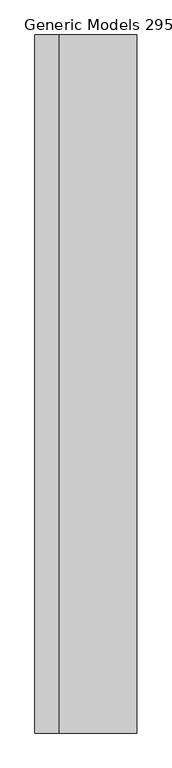
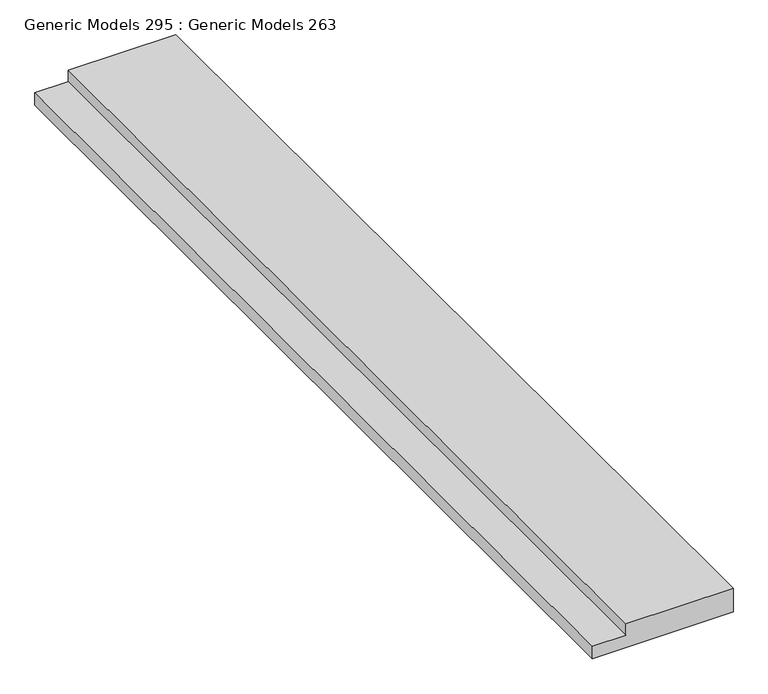
"""IFC4 building model written with IfcOpenShell, lengths in millimetres: proxy geometry, Generic Models 295 : Generic Models 263."""

import ifcopenshell
import ifcopenshell.guid

model = None  # the IFC model being written
_history = None  # IfcOwnerHistory: only IFC2X3 demands one
_inside = {}  # id of a spatial element -> (the spatial element, [elements in it])
_under = {}  # id of a project, library or spatial element -> (it, [spatial elements below it])
_declared = {}  # id of a project -> (the project, [libraries it declares])
_typed = {}  # id of a type object -> (the type object, [elements of that type])
_made_of = {}  # id of a material, layer set ... -> (it, [elements and type objects made of it])


def new_model(schema):
    """Start an empty IFC model of exactly this schema.

    Asked for "IFC4X3", IfcOpenShell would pick the latest addendum, in which some entities
    have other attributes; the version numbers below select the first issue.
    IFC2X3 requires an IfcOwnerHistory on every rooted entity: one is made here for all.
    """
    global model, _history
    if schema == "IFC4X3":
        model = ifcopenshell.file(schema_version=(4, 3, 0, 0))
    else:
        model = ifcopenshell.file(schema=schema)
    _inside.clear()
    _under.clear()
    _declared.clear()
    _typed.clear()
    _made_of.clear()
    _history = None
    if model.schema == "IFC2X3":
        org = make("IfcOrganization", Name="unknown")
        user = make(
            "IfcPersonAndOrganization",
            ThePerson=make("IfcPerson", FamilyName="unknown"),
            TheOrganization=org,
        )
        app = make(
            "IfcApplication",
            ApplicationDeveloper=org,
            Version="unknown",
            ApplicationFullName="unknown",
            ApplicationIdentifier="unknown",
        )
        _history = make(
            "IfcOwnerHistory",
            OwningUser=user,
            OwningApplication=app,
            ChangeAction="ADDED",
            CreationDate=0,
        )
    return model


def make(cls, **values):
    """One entity of the class cls with the attributes given. An attribute that is None is left unset."""
    return model.create_entity(
        cls, **{name: value for name, value in values.items() if value is not None}
    )


def rooted(cls, **values):
    """An entity with a GlobalId (a new one), such as an element, a storey or a relation."""
    return make(cls, GlobalId=ifcopenshell.guid.new(), OwnerHistory=_history, **values)


def si_unit(unit_type, name, prefix=None):
    """IfcSIUnit, for example si_unit("LENGTHUNIT", "METRE", prefix="MILLI")."""
    return make("IfcSIUnit", UnitType=unit_type, Prefix=prefix, Name=name)


def assignment(units):
    """IfcUnitAssignment: the units of a project."""
    return None if units is None else make("IfcUnitAssignment", Units=units)


def point(xyz):
    """IfcCartesianPoint."""
    return None if xyz is None else make("IfcCartesianPoint", Coordinates=xyz)


def direction(xyz):
    """IfcDirection."""
    return None if xyz is None else make("IfcDirection", DirectionRatios=xyz)


def frame(location, z_axis=None, x_axis=None):
    """IfcAxis2Placement3D, a coordinate frame: its origin and axes. An axis left out is left unset."""
    return make(
        "IfcAxis2Placement3D",
        Location=point(location),
        Axis=direction(z_axis),
        RefDirection=direction(x_axis),
    )


def origin():
    """The frame at (0, 0, 0) with its axes left unset."""
    return frame((0.0, 0.0, 0.0))


def place(relative_to, where):
    """IfcLocalPlacement: puts the frame where relative to a parent placement (None: the world)."""
    return make(
        "IfcLocalPlacement", PlacementRelTo=relative_to, RelativePlacement=where
    )


def context(
    kind, dimensions, precision=None, world=None, true_north=None, identifier=None
):
    """IfcGeometricRepresentationContext, for example the 3D "Model" context."""
    return make(
        "IfcGeometricRepresentationContext",
        ContextIdentifier=identifier,
        ContextType=kind,
        CoordinateSpaceDimension=dimensions,
        Precision=precision,
        WorldCoordinateSystem=world,
        TrueNorth=true_north,
    )


def project(units=None, contexts=None):
    """IfcProject with its units and contexts."""
    return rooted(
        "IfcProject",
        Name="project",
        RepresentationContexts=contexts,
        UnitsInContext=assignment(units),
    )


def spatial(cls, under=None, at=None, **own):
    """A site, building, storey or space (cls), placed at a placement, below another one or the project."""
    s = rooted(cls, ObjectPlacement=at, **own)
    if under is not None:
        _under.setdefault(under.id(), (under, []))[1].append(s)
    return s


def polyline(points):
    """IfcPolyline through the points."""
    return make("IfcPolyline", Points=[point(p) for p in points])


def outline(outer, holes=None, kind="AREA"):
    """IfcArbitraryClosedProfileDef: a profile drawn as a closed curve; with holes, ...WithVoids."""
    if holes is None:
        return make("IfcArbitraryClosedProfileDef", ProfileType=kind, OuterCurve=outer)
    return make(
        "IfcArbitraryProfileDefWithVoids",
        ProfileType=kind,
        OuterCurve=outer,
        InnerCurves=holes,
    )


def extrude(swept, where, along, depth):
    """IfcExtrudedAreaSolid: the profile swept, set in the frame where, extruded along a direction by depth."""
    return make(
        "IfcExtrudedAreaSolid",
        SweptArea=swept,
        Position=where,
        ExtrudedDirection=direction(along),
        Depth=depth,
    )


def shape(context_of_items, identifier, shape_type, items):
    """IfcShapeRepresentation: the items that make up one representation, for example the "Body"."""
    return make(
        "IfcShapeRepresentation",
        ContextOfItems=context_of_items,
        RepresentationIdentifier=identifier,
        RepresentationType=shape_type,
        Items=items,
    )


def source(mapping_origin, context_of_items, identifier, shape_type, items):
    """IfcRepresentationMap: a shape defined once, which mapped items show again and again."""
    return make(
        "IfcRepresentationMap",
        MappingOrigin=mapping_origin,
        MappedRepresentation=shape(context_of_items, identifier, shape_type, items),
    )


def transform(
    local_origin,
    x_axis=None,
    y_axis=None,
    z_axis=None,
    scale=None,
    scale2=None,
    scale3=None,
    uniform=True,
):
    """IfcCartesianTransformationOperator3D, or its non-uniform kind. x_axis, y_axis, z_axis: its Axis1, 2, 3."""
    if uniform:
        return make(
            "IfcCartesianTransformationOperator3D",
            Axis1=direction(x_axis),
            Axis2=direction(y_axis),
            LocalOrigin=point(local_origin),
            Scale=scale,
            Axis3=direction(z_axis),
        )
    return make(
        "IfcCartesianTransformationOperator3DnonUniform",
        Axis1=direction(x_axis),
        Axis2=direction(y_axis),
        LocalOrigin=point(local_origin),
        Scale=scale,
        Axis3=direction(z_axis),
        Scale2=scale2,
        Scale3=scale3,
    )


def mapped(mapping_source, mapping_target):
    """IfcMappedItem: shows the shape of a source again, moved by a transform."""
    return make(
        "IfcMappedItem", MappingSource=mapping_source, MappingTarget=mapping_target
    )


def made_of(thing, what):
    """Note that an element or type object is made of a material, layer set ...; save() writes the relation."""
    if what is not None:
        _made_of.setdefault(what.id(), (what, []))[1].append(thing)
    return thing


def element(
    cls,
    number,
    at=None,
    inside=None,
    cuts=None,
    type_object=None,
    material=None,
    context=None,
    identifier="Body",
    shape_type=None,
    held_by="IfcProductDefinitionShape",
    body=None,
    shapes=None,
    **own,
):
    """One element of the class cls, such as IfcWall. Its Tag is "e" and its number.

    at: its placement. inside: the storey or other place that contains it. cuts: it is an
    opening in that element (IfcRelVoidsElement). A single representation is given by context,
    identifier, shape_type and body (its items); several are given by shapes. held_by: the class
    of the entity that holds the representations. save() writes the other relations.
    """
    e = rooted(cls, Tag="e%d" % number, ObjectPlacement=at, **own)
    if body is not None:
        shapes = [shape(context, identifier, shape_type, body)]
    if shapes is not None:
        e.Representation = make(held_by, Representations=shapes)
    if inside is not None:
        _inside.setdefault(inside.id(), (inside, []))[1].append(e)
    if cuts is not None:
        rooted(
            "IfcRelVoidsElement", RelatingBuildingElement=cuts, RelatedOpeningElement=e
        )
    if type_object is not None:
        _typed.setdefault(type_object.id(), (type_object, []))[1].append(e)
    return made_of(e, material)


def aggregate(whole, parts):
    """IfcRelAggregates: a whole, such as a stair, and the parts it consists of."""
    return rooted("IfcRelAggregates", RelatingObject=whole, RelatedObjects=parts)


def save(model, path):
    """Write the relations noted so far, then the file.

    IfcRelAggregates (storeys below a building ...), IfcRelContainedInSpatialStructure (elements
    in a storey), IfcRelDefinesByType, IfcRelAssociatesMaterial and IfcRelDeclares: one each for
    every whole, place, type object, material and project.
    """
    for whole, parts in _under.values():
        aggregate(whole, parts)
    for where, things in _inside.values():
        rooted(
            "IfcRelContainedInSpatialStructure",
            RelatedElements=things,
            RelatingStructure=where,
        )
    for kind, things in _typed.values():
        rooted("IfcRelDefinesByType", RelatedObjects=things, RelatingType=kind)
    for what, things in _made_of.values():
        rooted("IfcRelAssociatesMaterial", RelatedObjects=things, RelatingMaterial=what)
    for by, libraries in _declared.values():
        rooted("IfcRelDeclares", RelatingContext=by, RelatedDefinitions=libraries)
    model.write(path)


def generic_models_295_generic_models_263_197a9b76(model_context):
    return source(origin(), model_context, "Body", "SweptSolid", [
        extrude(outline(polyline([(-381.0, 92037.1797726), (-381.0, 91579.9797726), (-558.8, 91579.9797726), (-558.8, 93498.3966125), (-215.9, 93498.3966125), (-215.9, 92037.1797726), (-381.0, 92037.1797726)])), frame((0.0, -4692.2809088, 0.0), z_axis=(0.0, 1.0, 0.0), x_axis=(0.0, 0.0, 1.0)), (0.0, 0.0, 1.0), 13158.0645094),
    ])


if __name__ == "__main__":
    model = new_model("IFC4")
    model_context = context("Model", 3, world=origin())
    ifc_project = project(units=[si_unit("LENGTHUNIT", "METRE", prefix="MILLI")], contexts=[model_context])
    site = spatial("IfcSite", under=ifc_project)
    building = spatial("IfcBuilding", under=site)
    placement = place(None, origin())
    generic_models_295_generic_models_263_shape = generic_models_295_generic_models_263_197a9b76(model_context)
    element("IfcBuildingElementProxy", 1, Name="Generic Models 295 : Generic Models 263", ObjectType="Generic Models 295 : Generic Models 263", at=placement, inside=building, context=model_context, shape_type="MappedRepresentation", body=[
        mapped(generic_models_295_generic_models_263_shape, transform((0.0, 0.0, 0.0), x_axis=(1.0, 0.0, 0.0), y_axis=(0.0, 1.0, 0.0), z_axis=(0.0, 0.0, 1.0))),
    ])
    save(model, "model.ifc")

# Revit data of these elements
# Element 1 (IfcBuildingElementProxy, "Generic Models 295 : Generic Models 263")
#   Materials on its faces: "CRUSHED AGGREGATE BASE COURSE"
# Materials
#   "CRUSHED AGGREGATE BASE COURSE": class "Miscellaneous", colour RGB 183 184 198, transparency 0, Cost = 0
